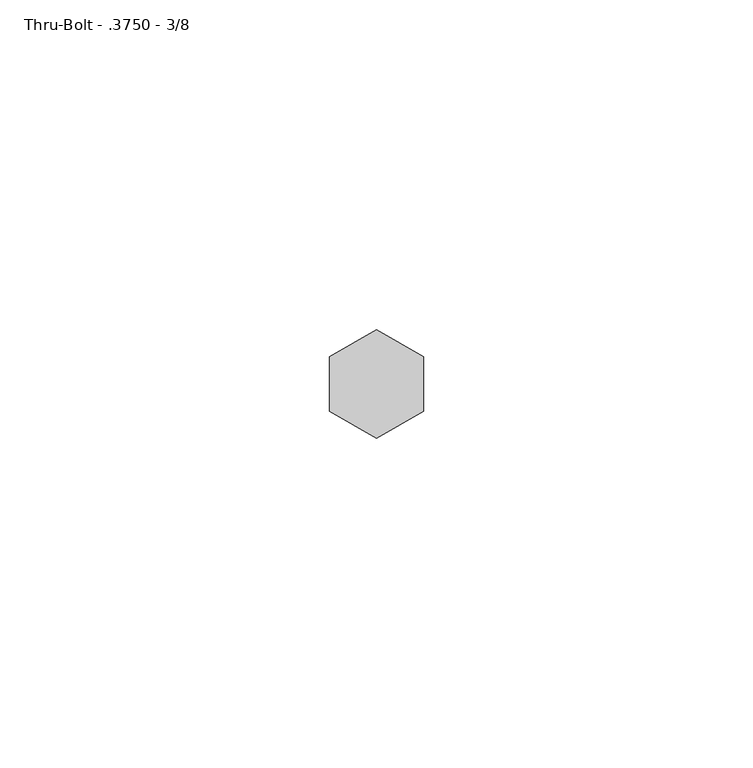
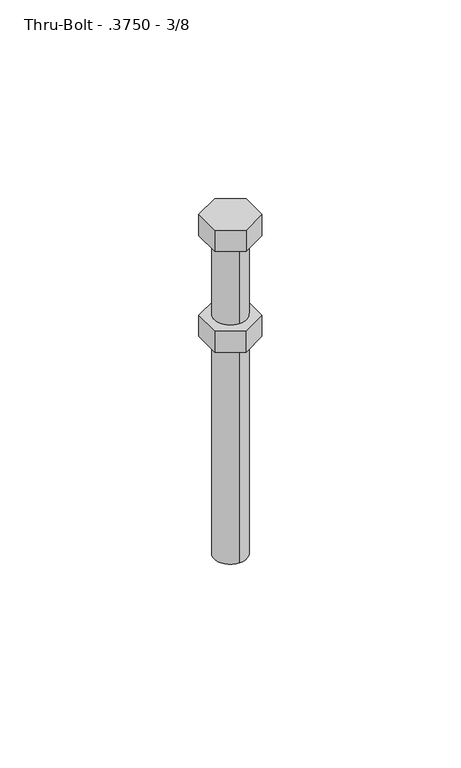
"""IFC4 building model written with IfcOpenShell, lengths in millimetres: fastener geometry, 060523 - W_P_C - Fastenings - Generic : Thru-Bolt - .3750 - 3/8."""

from ifc_helpers import new_model, si_unit, point, frame, origin, origin_with_axes, origin_2d, place, context, project, spatial, polyline, circle_curve, trimmed, segment, composite_curve, outline, extrude, source, transform, mapped, element, save


def thru_bolt_3750_3_8_3860eeba(model_context):
    return source(origin(), model_context, "Body", "SweptSolid", [
        extrude(outline(polyline([(-7.14375, -4.124446), (-7.14375, 4.124446), (0.0, 8.248892), (7.14375, 4.124446), (7.14375, -4.124446), (0.0, -8.248892), (-7.14375, -4.124446)])), frame((0.0, 0.0, -32.2072), z_axis=(0.0, 0.0, 1.0), x_axis=(1.0, 0.0, 0.0)), (0.0, 0.0, 1.0), 6.8072),
        extrude(outline(polyline([(-7.14375, 4.124446), (0.0, 8.248892), (7.14375, 4.124446), (7.14375, -4.124446), (0.0, -8.248892), (-7.14375, -4.124446), (-7.14375, 4.124446)])), origin_with_axes(), (0.0, 0.0, 1.0), 6.8072),
        extrude(outline(composite_curve([segment(trimmed(circle_curve(origin_2d(), 4.9113281), [point((0.0, -4.9113281))], [point((0.0, 4.9113281))], False, "CARTESIAN"), True, "CONTINUOUS"), segment(trimmed(circle_curve(origin_2d(), 4.9113281), [point((0.0, 4.9113281))], [point((0.0, -4.9113281))], False, "CARTESIAN"), True, "CONTINUOUS")], self_intersect=False)), frame((0.0, 0.0, -101.6), z_axis=(0.0, 0.0, 1.0), x_axis=(1.0, 0.0, 0.0)), (0.0, 0.0, 1.0), 101.6),
    ])


if __name__ == "__main__":
    model = new_model("IFC4")
    model_context = context("Model", 3, world=origin())
    ifc_project = project(units=[si_unit("LENGTHUNIT", "METRE", prefix="MILLI")], contexts=[model_context])
    site = spatial("IfcSite", under=ifc_project)
    building = spatial("IfcBuilding", under=site)
    placement = place(None, origin())
    thru_bolt_3750_3_8_shape = thru_bolt_3750_3_8_3860eeba(model_context)
    element("IfcFastener", 1, ObjectType="060523 - W_P_C - Fastenings - Generic : Thru-Bolt - .3750 - 3/8", at=placement, inside=building, context=model_context, shape_type="MappedRepresentation", body=[
        mapped(thru_bolt_3750_3_8_shape, transform((0.0, 0.0, 0.0), x_axis=(1.0, 0.0, 0.0), y_axis=(0.0, 1.0, 0.0), z_axis=(0.0, 0.0, 1.0))),
    ])
    save(model, "model.ifc")

# Revit data of these elements
# Type "060523 - W_P_C - Fastenings - Generic : Thru-Bolt - .3750 - 3/8"
#   Washer_Thickness = 0' - 0.08933"
#   Washer Radius = 0' - 0.46136"
#   Washer Offset - Head = 0' - 0"
#   Washer Offset = 0' - 0"
#   Thickness_of_Substrate [instance default] = 0' - 1"
#   Side = 0' - 0.3252"
#   Radius = 0' - 0.19336"
#   Length [instance default] = 0' - 4"
#   Head Size = 0' - 0 9/16"
#   Head Radius = 0' - 0 9/32"
#   Head Height = 0' - 0.268"
#   Double Diameter = 0' - 0 99/128"
#   Diameter = 0' - 0 99/256"
#   Default Elevation = 4' - 0"
#   Washer_Nut_Visibility = no
#   Washer_Head_Visibility = no
#   Round_Head_Visibility = no
#   Point Visibility = no
#   Nut_Visibility = yes
#   Hex_Head_Visiblilty = yes
#   Washer Material = none
#   Bolt Material (Size) = AT SILL - FASTENER AT 24" O.C.
# Element 1 (IfcFastener, "060523 - W_P_C - Fastenings - Generic : Thru-Bolt - .3750 - 3/8")
#   Materials on its faces: "AT SILL - FASTENER AT 24\" O.C."
# Materials
#   "AT SILL - FASTENER AT 24\" O.C.": class "Generic", colour RGB 120 120 120, transparency 0, Cost = 0
